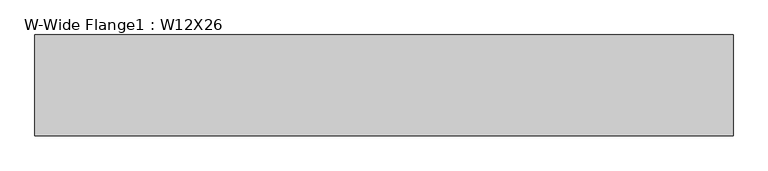
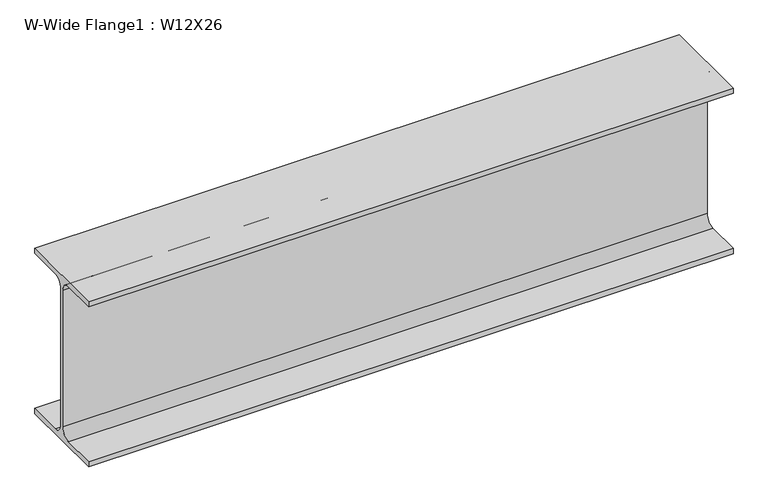
"""IFC4 building model written with IfcOpenShell, lengths in millimetres: beam geometry, W-Wide Flange1 : W12X26."""

from ifc_helpers import new_model, si_unit, point, frame, frame_2d, origin, place, context, project, spatial, polyline, circle_curve, trimmed, segment, composite_curve, outline, extrude, source, transform, mapped, element, save


def w_wide_flange1_w12x26_284a29d7(model_context):
    return source(origin(), model_context, "Body", "SweptSolid", [
        extrude(outline(composite_curve([segment(polyline([(82.423, -145.288), (82.423, -154.94), (-82.423, -154.94), (-82.423, -145.288), (-20.2565, -145.288)]), True, "CONTINUOUS"), segment(trimmed(circle_curve(frame_2d((-20.2565, -127.9525)), 17.3355), [point((-20.2565, -145.288))], [point((-2.921, -127.9525))], True, "CARTESIAN"), True, "CONTINUOUS"), segment(polyline([(-2.921, -127.9525), (-2.921, 127.9525)]), True, "CONTINUOUS"), segment(trimmed(circle_curve(frame_2d((-20.2565, 127.9525)), 17.3355), [point((-2.921, 127.9525))], [point((-20.2565, 145.288))], True, "CARTESIAN"), True, "CONTINUOUS"), segment(polyline([(-20.2565, 145.288), (-82.423, 145.288), (-82.423, 154.94), (82.423, 154.94), (82.423, 145.288), (20.2565, 145.288)]), True, "CONTINUOUS"), segment(trimmed(circle_curve(frame_2d((20.2565, 127.9525)), 17.3355), [point((20.2565, 145.288))], [point((2.921, 127.9525))], True, "CARTESIAN"), True, "CONTINUOUS"), segment(polyline([(2.921, 127.9525), (2.921, -127.9525)]), True, "CONTINUOUS"), segment(trimmed(circle_curve(frame_2d((20.2565, -127.9525)), 17.3355), [point((2.921, -127.9525))], [point((20.2565, -145.288))], True, "CARTESIAN"), True, "CONTINUOUS"), segment(polyline([(20.2565, -145.288), (82.423, -145.288)]), True, "CONTINUOUS")], self_intersect=False)), frame((-549.7694137, 0.0, 0.0), z_axis=(1.0, 0.0, 0.0), x_axis=(0.0, 1.0, 0.0)), (0.0, 0.0, 1.0), 1142.9822398),
    ])


if __name__ == "__main__":
    model = new_model("IFC4")
    model_context = context("Model", 3, world=origin())
    ifc_project = project(units=[si_unit("LENGTHUNIT", "METRE", prefix="MILLI")], contexts=[model_context])
    site = spatial("IfcSite", under=ifc_project)
    building = spatial("IfcBuilding", under=site)
    placement = place(None, origin())
    w_wide_flange1_w12x26_shape = w_wide_flange1_w12x26_284a29d7(model_context)
    element("IfcBeam", 1, ObjectType="W-Wide Flange1 : W12X26", at=placement, inside=building, context=model_context, shape_type="MappedRepresentation", body=[
        mapped(w_wide_flange1_w12x26_shape, transform((0.0, 0.0, 0.0), x_axis=(1.0, 0.0, 0.0), y_axis=(0.0, 1.0, 0.0), z_axis=(0.0, 0.0, 1.0))),
    ])
    save(model, "model.ifc")

# Revit data of these elements
# Type "W-Wide Flange1 : W12X26"
#   Assembly Code = "B10"
#   W = 26
#   Start Extension Calculation [instance default] = 10' - 0"
#   Start Extension [instance default] = -0' - 0 1/2"
#   End Extension Calculation [instance default] = 10' - 0"
#   End Extension [instance default] = -0' - 0 1/2"
#   Length [instance default] = 5' - 0"
#   bf = 0' - 6.49"
#   d = 1' - 0.2"
#   k = 0' - 1 1/16"
#   k2 = 0' - 0.6825"
#   tf = 0' - 0.38"
#   tw = 0' - 0.23"
#   A = 0.053125 SF
#   Structural Material [instance default] = Metal - Steel - ASTM A992
# Element 1 (IfcBeam, "W-Wide Flange1 : W12X26")
#   Materials on its faces: "Metal - Steel - ASTM A992"
# Materials
#   "Metal - Steel - ASTM A992": class "Metal", colour RGB 199 199 199, transparency 0
